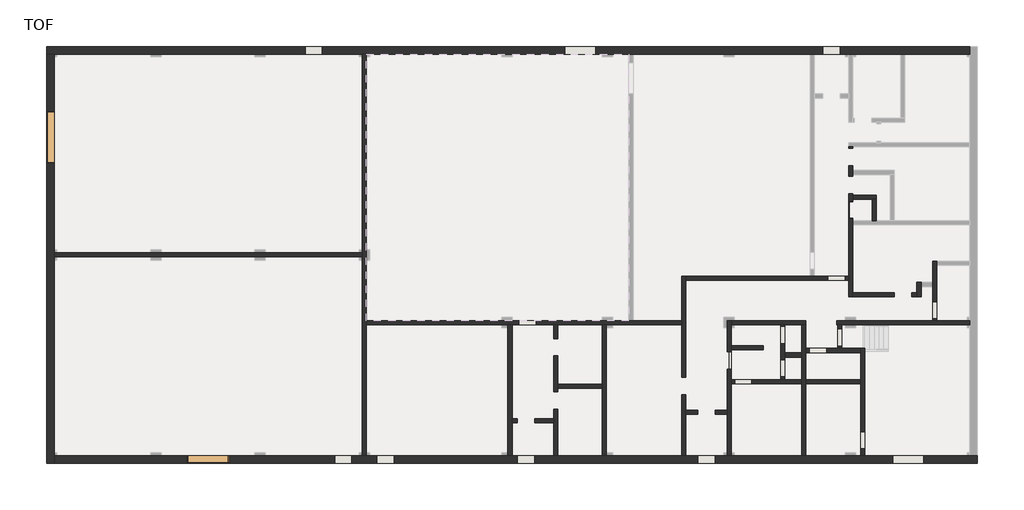
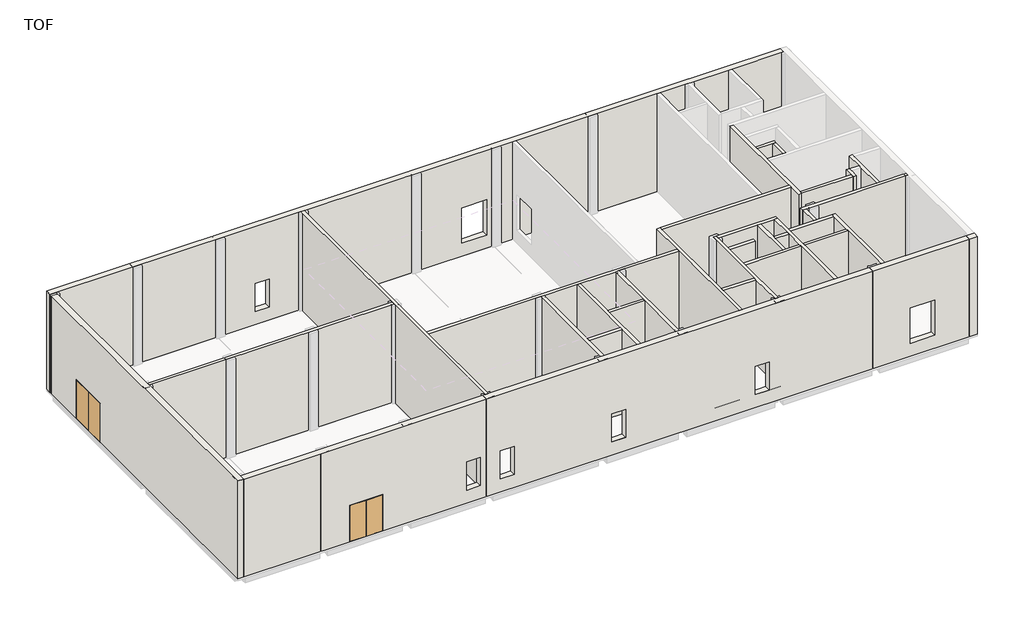
# One storey, part 1 of 3: 31 walls, 3 doors.
"""IFC4 building model written with IfcOpenShell, lengths in millimetres."""

import ifcopenshell
import ifcopenshell.guid

model = None  # the IFC model being written
_history = None  # IfcOwnerHistory: only IFC2X3 demands one
_inside = {}  # id of a spatial element -> (the spatial element, [elements in it])
_under = {}  # id of a project, library or spatial element -> (it, [spatial elements below it])
_declared = {}  # id of a project -> (the project, [libraries it declares])
_typed = {}  # id of a type object -> (the type object, [elements of that type])
_made_of = {}  # id of a material, layer set ... -> (it, [elements and type objects made of it])


def new_model(schema):
    """Start an empty IFC model of exactly this schema.

    Asked for "IFC4X3", IfcOpenShell would pick the latest addendum, in which some entities
    have other attributes; the version numbers below select the first issue.
    IFC2X3 requires an IfcOwnerHistory on every rooted entity: one is made here for all.
    """
    global model, _history
    if schema == "IFC4X3":
        model = ifcopenshell.file(schema_version=(4, 3, 0, 0))
    else:
        model = ifcopenshell.file(schema=schema)
    _inside.clear()
    _under.clear()
    _declared.clear()
    _typed.clear()
    _made_of.clear()
    _history = None
    if model.schema == "IFC2X3":
        org = make("IfcOrganization", Name="unknown")
        user = make(
            "IfcPersonAndOrganization",
            ThePerson=make("IfcPerson", FamilyName="unknown"),
            TheOrganization=org,
        )
        app = make(
            "IfcApplication",
            ApplicationDeveloper=org,
            Version="unknown",
            ApplicationFullName="unknown",
            ApplicationIdentifier="unknown",
        )
        _history = make(
            "IfcOwnerHistory",
            OwningUser=user,
            OwningApplication=app,
            ChangeAction="ADDED",
            CreationDate=0,
        )
    return model


def make(cls, **values):
    """One entity of the class cls with the attributes given. An attribute that is None is left unset."""
    return model.create_entity(
        cls, **{name: value for name, value in values.items() if value is not None}
    )


def rooted(cls, **values):
    """An entity with a GlobalId (a new one), such as an element, a storey or a relation."""
    return make(cls, GlobalId=ifcopenshell.guid.new(), OwnerHistory=_history, **values)


def si_unit(unit_type, name, prefix=None):
    """IfcSIUnit, for example si_unit("LENGTHUNIT", "METRE", prefix="MILLI")."""
    return make("IfcSIUnit", UnitType=unit_type, Prefix=prefix, Name=name)


def assignment(units):
    """IfcUnitAssignment: the units of a project."""
    return None if units is None else make("IfcUnitAssignment", Units=units)


def point(xyz):
    """IfcCartesianPoint."""
    return None if xyz is None else make("IfcCartesianPoint", Coordinates=xyz)


def direction(xyz):
    """IfcDirection."""
    return None if xyz is None else make("IfcDirection", DirectionRatios=xyz)


def frame(location, z_axis=None, x_axis=None):
    """IfcAxis2Placement3D, a coordinate frame: its origin and axes. An axis left out is left unset."""
    return make(
        "IfcAxis2Placement3D",
        Location=point(location),
        Axis=direction(z_axis),
        RefDirection=direction(x_axis),
    )


def origin():
    """The frame at (0, 0, 0) with its axes left unset."""
    return frame((0.0, 0.0, 0.0))


def place(relative_to, where):
    """IfcLocalPlacement: puts the frame where relative to a parent placement (None: the world)."""
    return make(
        "IfcLocalPlacement", PlacementRelTo=relative_to, RelativePlacement=where
    )


def context(
    kind, dimensions, precision=None, world=None, true_north=None, identifier=None
):
    """IfcGeometricRepresentationContext, for example the 3D "Model" context."""
    return make(
        "IfcGeometricRepresentationContext",
        ContextIdentifier=identifier,
        ContextType=kind,
        CoordinateSpaceDimension=dimensions,
        Precision=precision,
        WorldCoordinateSystem=world,
        TrueNorth=true_north,
    )


def project(units=None, contexts=None):
    """IfcProject with its units and contexts."""
    return rooted(
        "IfcProject",
        Name="project",
        RepresentationContexts=contexts,
        UnitsInContext=assignment(units),
    )


def spatial(cls, under=None, at=None, **own):
    """A site, building, storey or space (cls), placed at a placement, below another one or the project."""
    s = rooted(cls, ObjectPlacement=at, **own)
    if under is not None:
        _under.setdefault(under.id(), (under, []))[1].append(s)
    return s


def polyline(points):
    """IfcPolyline through the points."""
    return make("IfcPolyline", Points=[point(p) for p in points])


def outline(outer, holes=None, kind="AREA"):
    """IfcArbitraryClosedProfileDef: a profile drawn as a closed curve; with holes, ...WithVoids."""
    if holes is None:
        return make("IfcArbitraryClosedProfileDef", ProfileType=kind, OuterCurve=outer)
    return make(
        "IfcArbitraryProfileDefWithVoids",
        ProfileType=kind,
        OuterCurve=outer,
        InnerCurves=holes,
    )


def extrude(swept, where, along, depth):
    """IfcExtrudedAreaSolid: the profile swept, set in the frame where, extruded along a direction by depth."""
    return make(
        "IfcExtrudedAreaSolid",
        SweptArea=swept,
        Position=where,
        ExtrudedDirection=direction(along),
        Depth=depth,
    )


def faces_of(points, faces, orient=None, outer=None):
    """IfcFace entities. A face is a list of loops; a loop is a list of indices into points, from 0.

    orient and outer hold one flag for each loop. By default every Orientation is true, the
    first loop of a face is its IfcFaceOuterBound and the others are IfcFaceBound.
    """
    made = []
    for i, loops in enumerate(faces):
        bounds = []
        for j, loop in enumerate(loops):
            is_outer = j == 0 if outer is None else outer[i][j]
            bounds.append(
                make(
                    "IfcFaceOuterBound" if is_outer else "IfcFaceBound",
                    Bound=make("IfcPolyLoop", Polygon=[points[k] for k in loop]),
                    Orientation=True if orient is None else orient[i][j],
                )
            )
        made.append(make("IfcFace", Bounds=bounds))
    return made


def faceted_brep(points, faces, orient=None, outer=None, voids=None):
    """IfcFacetedBrep: a solid bounded by flat faces; with voids (closed shells), ...WithVoids."""
    shared = [point(p) for p in points]
    hull = make("IfcClosedShell", CfsFaces=faces_of(shared, faces, orient, outer))
    if voids is None:
        return make("IfcFacetedBrep", Outer=hull)
    return make(
        "IfcFacetedBrepWithVoids",
        Outer=hull,
        Voids=[
            make(cls, CfsFaces=faces_of(shared, fs, o, b)) for cls, fs, o, b in voids
        ],
    )


def shape(context_of_items, identifier, shape_type, items):
    """IfcShapeRepresentation: the items that make up one representation, for example the "Body"."""
    return make(
        "IfcShapeRepresentation",
        ContextOfItems=context_of_items,
        RepresentationIdentifier=identifier,
        RepresentationType=shape_type,
        Items=items,
    )


def source(mapping_origin, context_of_items, identifier, shape_type, items):
    """IfcRepresentationMap: a shape defined once, which mapped items show again and again."""
    return make(
        "IfcRepresentationMap",
        MappingOrigin=mapping_origin,
        MappedRepresentation=shape(context_of_items, identifier, shape_type, items),
    )


def transform(
    local_origin,
    x_axis=None,
    y_axis=None,
    z_axis=None,
    scale=None,
    scale2=None,
    scale3=None,
    uniform=True,
):
    """IfcCartesianTransformationOperator3D, or its non-uniform kind. x_axis, y_axis, z_axis: its Axis1, 2, 3."""
    if uniform:
        return make(
            "IfcCartesianTransformationOperator3D",
            Axis1=direction(x_axis),
            Axis2=direction(y_axis),
            LocalOrigin=point(local_origin),
            Scale=scale,
            Axis3=direction(z_axis),
        )
    return make(
        "IfcCartesianTransformationOperator3DnonUniform",
        Axis1=direction(x_axis),
        Axis2=direction(y_axis),
        LocalOrigin=point(local_origin),
        Scale=scale,
        Axis3=direction(z_axis),
        Scale2=scale2,
        Scale3=scale3,
    )


def mapped(mapping_source, mapping_target):
    """IfcMappedItem: shows the shape of a source again, moved by a transform."""
    return make(
        "IfcMappedItem", MappingSource=mapping_source, MappingTarget=mapping_target
    )


def made_of(thing, what):
    """Note that an element or type object is made of a material, layer set ...; save() writes the relation."""
    if what is not None:
        _made_of.setdefault(what.id(), (what, []))[1].append(thing)
    return thing


def element(
    cls,
    number,
    at=None,
    inside=None,
    cuts=None,
    type_object=None,
    material=None,
    context=None,
    identifier="Body",
    shape_type=None,
    held_by="IfcProductDefinitionShape",
    body=None,
    shapes=None,
    **own,
):
    """One element of the class cls, such as IfcWall. Its Tag is "e" and its number.

    at: its placement. inside: the storey or other place that contains it. cuts: it is an
    opening in that element (IfcRelVoidsElement). A single representation is given by context,
    identifier, shape_type and body (its items); several are given by shapes. held_by: the class
    of the entity that holds the representations. save() writes the other relations.
    """
    e = rooted(cls, Tag="e%d" % number, ObjectPlacement=at, **own)
    if body is not None:
        shapes = [shape(context, identifier, shape_type, body)]
    if shapes is not None:
        e.Representation = make(held_by, Representations=shapes)
    if inside is not None:
        _inside.setdefault(inside.id(), (inside, []))[1].append(e)
    if cuts is not None:
        rooted(
            "IfcRelVoidsElement", RelatingBuildingElement=cuts, RelatedOpeningElement=e
        )
    if type_object is not None:
        _typed.setdefault(type_object.id(), (type_object, []))[1].append(e)
    return made_of(e, material)


def aggregate(whole, parts):
    """IfcRelAggregates: a whole, such as a stair, and the parts it consists of."""
    return rooted("IfcRelAggregates", RelatingObject=whole, RelatedObjects=parts)


def save(model, path):
    """Write the relations noted so far, then the file.

    IfcRelAggregates (storeys below a building ...), IfcRelContainedInSpatialStructure (elements
    in a storey), IfcRelDefinesByType, IfcRelAssociatesMaterial and IfcRelDeclares: one each for
    every whole, place, type object, material and project.
    """
    for whole, parts in _under.values():
        aggregate(whole, parts)
    for where, things in _inside.values():
        rooted(
            "IfcRelContainedInSpatialStructure",
            RelatedElements=things,
            RelatingStructure=where,
        )
    for kind, things in _typed.values():
        rooted("IfcRelDefinesByType", RelatedObjects=things, RelatingType=kind)
    for what, things in _made_of.values():
        rooted("IfcRelAssociatesMaterial", RelatedObjects=things, RelatingMaterial=what)
    for by, libraries in _declared.values():
        rooted("IfcRelDeclares", RelatingContext=by, RelatedDefinitions=libraries)
    model.write(path)


def double_door_steel_89dfd0fe(model_context):
    return source(origin(), model_context, "Body", "SolidModel", [
        extrude(outline(polyline([(1480.0, 175.0), (0.0, 175.0), (0.0, 215.0), (1480.0, 215.0), (1480.0, 175.0)])), frame((0.0, 0.0, 20.0), z_axis=(0.0, 0.0, 1.0), x_axis=(1.0, 0.0, 0.0)), (0.0, 0.0, 1.0), 2960.0),
        extrude(outline(polyline([(0.0, 175.0), (-1480.0, 175.0), (-1480.0, 215.0), (0.0, 215.0), (0.0, 175.0)])), frame((0.0, 0.0, 20.0), z_axis=(0.0, 0.0, 1.0), x_axis=(1.0, 0.0, 0.0)), (0.0, 0.0, 1.0), 2960.0),
        faceted_brep([(1500.0, -215.0, 3000.0), (1500.0, 215.0, 3000.0), (-1500.0, 215.0, 3000.0), (-1500.0, -215.0, 3000.0), (1465.0, 175.0, 2965.0), (1465.0, -215.0, 2965.0), (-1465.0, -215.0, 2965.0), (-1465.0, 175.0, 2965.0), (1480.0, 215.0, 2980.0), (1480.0, 175.0, 2980.0), (-1480.0, 175.0, 2980.0), (-1480.0, 215.0, 2980.0), (-1500.0, 215.0, 0.0), (-1500.0, -215.0, 0.0), (-1465.0, -215.0, 35.0), (-1465.0, 175.0, 35.0), (-1480.0, 175.0, 20.0), (-1480.0, 215.0, 20.0), (1500.0, 215.0, 0.0), (1480.0, 215.0, 20.0), (1500.0, -215.0, 0.0), (1465.0, -215.0, 35.0), (1465.0, 175.0, 35.0), (1480.0, 175.0, 20.0)], [[[0, 1, 2, 3]], [[4, 5, 6, 7]], [[8, 9, 10, 11]], [[3, 2, 12, 13]], [[7, 6, 14, 15]], [[11, 10, 16, 17]], [[18, 12, 2, 1], [8, 11, 17, 19]], [[13, 12, 18, 20]], [[0, 3, 13, 20], [21, 14, 6, 5]], [[15, 14, 21, 22]], [[23, 16, 10, 9], [4, 7, 15, 22]], [[17, 16, 23, 19]], [[20, 18, 1, 0]], [[22, 21, 5, 4]], [[19, 23, 9, 8]]]),
    ])


def double_door_steel_f76c4a76(model_context):
    return source(origin(), model_context, "Body", "SolidModel", [
        extrude(outline(polyline([(1180.0, 175.0), (0.0, 175.0), (0.0, 215.0), (1180.0, 215.0), (1180.0, 175.0)])), frame((0.0, 0.0, 20.0), z_axis=(0.0, 0.0, 1.0), x_axis=(1.0, 0.0, 0.0)), (0.0, 0.0, 1.0), 2760.0),
        extrude(outline(polyline([(0.0, 175.0), (-1180.0, 175.0), (-1180.0, 215.0), (0.0, 215.0), (0.0, 175.0)])), frame((0.0, 0.0, 20.0), z_axis=(0.0, 0.0, 1.0), x_axis=(1.0, 0.0, 0.0)), (0.0, 0.0, 1.0), 2760.0),
        faceted_brep([(1200.0, -215.0, 0.0), (1200.0, 215.0, 0.0), (1200.0, 215.0, 2800.0), (1200.0, -215.0, 2800.0), (-1200.0, 215.0, 2800.0), (-1200.0, -215.0, 2800.0), (-1200.0, 215.0, 0.0), (1180.0, 215.0, 2780.0), (-1180.0, 215.0, 2780.0), (-1180.0, 215.0, 20.0), (1180.0, 215.0, 20.0), (-1200.0, -215.0, 0.0), (1165.0, -215.0, 35.0), (-1165.0, -215.0, 35.0), (-1165.0, -215.0, 2765.0), (1165.0, -215.0, 2765.0), (1165.0, 175.0, 35.0), (1165.0, 175.0, 2765.0), (-1165.0, 175.0, 2765.0), (-1165.0, 175.0, 35.0), (1180.0, 175.0, 20.0), (-1180.0, 175.0, 20.0), (-1180.0, 175.0, 2780.0), (1180.0, 175.0, 2780.0)], [[[0, 1, 2, 3]], [[3, 2, 4, 5]], [[1, 6, 4, 2], [7, 8, 9, 10]], [[5, 4, 6, 11]], [[3, 5, 11, 0], [12, 13, 14, 15]], [[16, 12, 15, 17]], [[17, 15, 14, 18]], [[18, 14, 13, 19]], [[20, 21, 22, 23], [17, 18, 19, 16]], [[10, 20, 23, 7]], [[7, 23, 22, 8]], [[8, 22, 21, 9]], [[11, 6, 1, 0]], [[19, 13, 12, 16]], [[9, 21, 20, 10]]]),
    ])


def double_door_steel_898613e4(model_context):
    return source(origin(), model_context, "Body", "SolidModel", [
        extrude(outline(polyline([(480.0, 77.0), (0.0, 77.0), (0.0, 117.0), (480.0, 117.0), (480.0, 77.0)])), frame((0.0, 0.0, 20.0), z_axis=(0.0, 0.0, 1.0), x_axis=(1.0, 0.0, 0.0)), (0.0, 0.0, 1.0), 2110.0),
        extrude(outline(polyline([(0.0, 77.0), (-480.0, 77.0), (-480.0, 117.0), (0.0, 117.0), (0.0, 77.0)])), frame((0.0, 0.0, 20.0), z_axis=(0.0, 0.0, 1.0), x_axis=(1.0, 0.0, 0.0)), (0.0, 0.0, 1.0), 2110.0),
        faceted_brep([(500.0, -117.0, 0.0), (500.0, 117.0, 0.0), (500.0, 117.0, 2150.0), (500.0, -117.0, 2150.0), (-500.0, 117.0, 2150.0), (-500.0, -117.0, 2150.0), (-500.0, 117.0, 0.0), (480.0, 117.0, 2130.0), (-480.0, 117.0, 2130.0), (-480.0, 117.0, 20.0), (480.0, 117.0, 20.0), (-500.0, -117.0, 0.0), (465.0, -117.0, 35.0), (-465.0, -117.0, 35.0), (-465.0, -117.0, 2115.0), (465.0, -117.0, 2115.0), (465.0, 77.0, 35.0), (465.0, 77.0, 2115.0), (-465.0, 77.0, 2115.0), (-465.0, 77.0, 35.0), (480.0, 77.0, 20.0), (-480.0, 77.0, 20.0), (-480.0, 77.0, 2130.0), (480.0, 77.0, 2130.0)], [[[0, 1, 2, 3]], [[3, 2, 4, 5]], [[1, 6, 4, 2], [7, 8, 9, 10]], [[5, 4, 6, 11]], [[3, 5, 11, 0], [12, 13, 14, 15]], [[16, 12, 15, 17]], [[17, 15, 14, 18]], [[18, 14, 13, 19]], [[20, 21, 22, 23], [17, 18, 19, 16]], [[10, 20, 23, 7]], [[7, 23, 22, 8]], [[8, 22, 21, 9]], [[11, 6, 1, 0]], [[19, 13, 12, 16]], [[9, 21, 20, 10]]]),
    ])


model = new_model("IFC4")

# Units and contexts
model_context = context("Model", 3, world=origin())
ifc_project = project(units=[si_unit("LENGTHUNIT", "METRE", prefix="MILLI")], contexts=[model_context])

# Site, building, storey
site = spatial("IfcSite", under=ifc_project)
building = spatial("IfcBuilding", under=site)
storey = spatial("IfcBuildingStorey", under=building, Name="TOF", Elevation=150.0)

# Doors
placement = place(None, origin())
double_door_steel_shape = double_door_steel_89dfd0fe(model_context)
element("IfcDoor", 1, ObjectType="Double Door_Steel : H_DR_AMB_Double Door_Steel_W3000xH3000", at=placement, inside=storey, context=model_context, shape_type="MappedRepresentation", body=[
    mapped(double_door_steel_shape, transform((-160.3, 19086.5208589, 150.0), x_axis=(0.0, 1.0, 0.0), y_axis=(-1.0, 0.0, 0.0), z_axis=(0.0, 0.0, 1.0))),
])
double_door_steel_2_shape = double_door_steel_f76c4a76(model_context)
element("IfcDoor", 2, ObjectType="Double Door_Steel : H_DR_AMB_Double Door_Steel_W2400xH2800", at=placement, inside=storey, context=model_context, shape_type="MappedRepresentation", body=[
    mapped(double_door_steel_2_shape, transform((8931.2, 531.5208589, 150.0), x_axis=(-1.0, 0.0, 0.0), y_axis=(0.0, -1.0, 0.0), z_axis=(0.0, 0.0, 1.0))),
])
double_door_steel_3_shape = double_door_steel_898613e4(model_context)
element("IfcDoor", 3, ObjectType="Double Door_Steel : H_DR_AMB_Double Door_Steel_W1000xH2150", at=placement, inside=storey, context=model_context, shape_type="MappedRepresentation", body=[
    mapped(double_door_steel_3_shape, transform((45924.7, 14901.8721317, 150.0), x_axis=(0.0, 1.0, 0.0), y_axis=(-1.0, 0.0, 0.0), z_axis=(0.0, 0.0, 1.0))),
])

# Walls
element("IfcWall", 4, ObjectType="H_WA_AMW_Brick Wall_Ext (0.5B_50_1.0B / Emulsion)", at=placement, inside=storey, context=model_context, shape_type="Brep", body=[
    faceted_brep([(-375.3, 23886.5208589, 150.0), (54.7, 23886.5208589, 150.0), (17807.7, 23886.5208589, 150.0), (18041.7, 23886.5208589, 150.0), (33157.7, 23886.5208589, 150.0), (33391.7, 23886.5208589, 150.0), (43607.7, 23886.5208589, 150.0), (43841.7, 23886.5208589, 150.0), (52794.7, 23886.5208589, 150.0), (52794.7, 23886.5208589, 7650.0), (49041.7, 23886.5208589, 7650.0), (48807.7, 23886.5208589, 7650.0), (46041.7, 23886.5208589, 7650.0), (45807.7, 23886.5208589, 7650.0), (43841.7, 23886.5208589, 7650.0), (43607.7, 23886.5208589, 7650.0), (33391.7, 23886.5208589, 7650.0), (33157.7, 23886.5208589, 7650.0), (18041.7, 23886.5208589, 7650.0), (17807.7, 23886.5208589, 7650.0), (54.7, 23886.5208589, 7650.0), (-375.3, 23886.5208589, 7650.0), (14507.7, 23886.5208589, 1150.0), (14507.7, 23886.5208589, 3300.0), (15507.7, 23886.5208589, 3300.0), (15507.7, 23886.5208589, 1150.0), (31257.7, 23886.5208589, 3850.0), (31257.7, 23886.5208589, 1150.0), (29457.7, 23886.5208589, 1150.0), (29457.7, 23886.5208589, 3850.0), (44324.7, 23886.5208589, 1150.0), (44324.7, 23886.5208589, 3300.0), (45324.7, 23886.5208589, 3300.0), (45324.7, 23886.5208589, 1150.0), (52794.7, 24316.5208589, 150.0), (-375.3, 24316.5208589, 150.0), (-375.3, 24316.5208589, 7650.0), (52794.7, 24316.5208589, 7650.0), (14507.7, 24316.5208589, 3300.0), (14507.7, 24316.5208589, 1150.0), (15507.7, 24316.5208589, 1150.0), (15507.7, 24316.5208589, 3300.0), (31257.7, 24316.5208589, 1150.0), (31257.7, 24316.5208589, 3850.0), (29457.7, 24316.5208589, 3850.0), (29457.7, 24316.5208589, 1150.0), (44324.7, 24316.5208589, 3300.0), (44324.7, 24316.5208589, 1150.0), (45324.7, 24316.5208589, 1150.0), (45324.7, 24316.5208589, 3300.0)], [[[0, 1, 2, 3, 4, 5, 6, 7, 8, 9, 10, 11, 12, 13, 14, 15, 16, 17, 18, 19, 20, 21], [22, 23, 24, 25], [26, 27, 28, 29], [30, 31, 32, 33]], [[34, 35, 36, 37], [38, 39, 40, 41], [42, 43, 44, 45], [46, 47, 48, 49]], [[8, 7, 6, 5, 4, 3, 2, 1, 0, 35, 34]], [[21, 20, 19, 18, 17, 16, 15, 14, 13, 12, 11, 10, 9, 37, 36]], [[0, 21, 36, 35]], [[9, 8, 34, 37]], [[22, 39, 38, 23]], [[23, 38, 41, 24]], [[24, 41, 40, 25]], [[39, 22, 25, 40]], [[42, 27, 26, 43]], [[43, 26, 29, 44]], [[28, 45, 44, 29]], [[27, 42, 45, 28]], [[31, 30, 47, 46]], [[32, 31, 46, 49]], [[33, 32, 49, 48]], [[30, 33, 48, 47]]]),
])
element("IfcWall", 5, ObjectType="H_WA_AMW_Brick Wall_Ext (0.5B_50_1.0B / Emulsion)", at=placement, inside=storey, context=model_context, shape_type="Brep", body=[
    faceted_brep([(54.7, 23886.5208589, 7650.0), (54.7, 12433.5208589, 7650.0), (54.7, 12199.5208589, 7650.0), (54.7, 746.5208589, 7650.0), (54.7, 316.5208589, 7650.0), (54.7, 316.5208589, 150.0), (54.7, 746.5208589, 150.0), (54.7, 12199.5208589, 150.0), (54.7, 12433.5208589, 150.0), (54.7, 17586.5208589, 150.0), (54.7, 17586.5208589, 3150.0), (54.7, 20586.5208589, 3150.0), (54.7, 20586.5208589, 150.0), (54.7, 23886.5208589, 150.0), (-375.3, 316.5208589, 7650.0), (-375.3, 23886.5208589, 7650.0), (-375.3, 23886.5208589, 150.0), (-375.3, 20586.5208589, 150.0), (-375.3, 20586.5208589, 3150.0), (-375.3, 17586.5208589, 3150.0), (-375.3, 17586.5208589, 150.0), (-375.3, 316.5208589, 150.0)], [[[0, 1, 2, 3, 4, 5, 6, 7, 8, 9, 10, 11, 12, 13]], [[14, 15, 16, 17, 18, 19, 20, 21]], [[5, 21, 20, 9, 8, 7, 6]], [[16, 13, 12, 17]], [[4, 3, 2, 1, 0, 15, 14]], [[5, 4, 14, 21]], [[0, 13, 16, 15]], [[11, 18, 17, 12]], [[18, 11, 10, 19]], [[19, 10, 9, 20]]]),
])
element("IfcWall", 6, ObjectType="H_WA_AMW_Brick Wall_Ext (0.5B_50_1.0B / Emulsion)", at=placement, inside=storey, context=model_context, shape_type="Brep", body=[
    faceted_brep([(54.7, 746.5208589, 7650.0), (17807.7, 746.5208589, 7650.0), (18041.7, 746.5208589, 7650.0), (26190.7, 746.5208589, 7650.0), (26424.7, 746.5208589, 7650.0), (28824.7, 746.5208589, 7650.0), (29058.7, 746.5208589, 7650.0), (31624.7, 746.5208589, 7650.0), (31858.7, 746.5208589, 7650.0), (36207.7, 746.5208589, 7650.0), (36441.7, 746.5208589, 7650.0), (38807.7, 746.5208589, 7650.0), (39041.7, 746.5208589, 7650.0), (43107.7, 746.5208589, 7650.0), (43341.7, 746.5208589, 7650.0), (46507.7, 746.5208589, 7650.0), (46741.7, 746.5208589, 7650.0), (52794.7, 746.5208589, 7650.0), (53224.7, 746.5208589, 7650.0), (53224.7, 746.5208589, 150.0), (52794.7, 746.5208589, 150.0), (46741.7, 746.5208589, 150.0), (46507.7, 746.5208589, 150.0), (43341.7, 746.5208589, 150.0), (43107.7, 746.5208589, 150.0), (39041.7, 746.5208589, 150.0), (38807.7, 746.5208589, 150.0), (26424.7, 746.5208589, 150.0), (26190.7, 746.5208589, 150.0), (18041.7, 746.5208589, 150.0), (17807.7, 746.5208589, 150.0), (10131.2, 746.5208589, 150.0), (10131.2, 746.5208589, 2950.0), (7731.2, 746.5208589, 2950.0), (7731.2, 746.5208589, 150.0), (54.7, 746.5208589, 150.0), (16207.7, 746.5208589, 3300.0), (16207.7, 746.5208589, 1150.0), (17207.7, 746.5208589, 1150.0), (17207.7, 746.5208589, 3300.0), (19641.7, 746.5208589, 1150.0), (19641.7, 746.5208589, 3300.0), (18641.7, 746.5208589, 3300.0), (18641.7, 746.5208589, 1150.0), (27724.7, 746.5208589, 1150.0), (27724.7, 746.5208589, 3300.0), (26724.7, 746.5208589, 3300.0), (26724.7, 746.5208589, 1150.0), (37124.7, 746.5208589, 3300.0), (37124.7, 746.5208589, 1150.0), (38124.7, 746.5208589, 1150.0), (38124.7, 746.5208589, 3300.0), (48341.7, 746.5208589, 3850.0), (48341.7, 746.5208589, 1150.0), (50141.7, 746.5208589, 1150.0), (50141.7, 746.5208589, 3850.0), (53224.7, 316.5208589, 7650.0), (54.7, 316.5208589, 7650.0), (54.7, 316.5208589, 150.0), (7731.2, 316.5208589, 150.0), (7731.2, 316.5208589, 2950.0), (10131.2, 316.5208589, 2950.0), (10131.2, 316.5208589, 150.0), (53224.7, 316.5208589, 150.0), (16207.7, 316.5208589, 1150.0), (16207.7, 316.5208589, 3300.0), (17207.7, 316.5208589, 3300.0), (17207.7, 316.5208589, 1150.0), (19641.7, 316.5208589, 3300.0), (19641.7, 316.5208589, 1150.0), (18641.7, 316.5208589, 1150.0), (18641.7, 316.5208589, 3300.0), (27724.7, 316.5208589, 3300.0), (27724.7, 316.5208589, 1150.0), (26724.7, 316.5208589, 1150.0), (26724.7, 316.5208589, 3300.0), (37124.7, 316.5208589, 1150.0), (37124.7, 316.5208589, 3300.0), (38124.7, 316.5208589, 3300.0), (38124.7, 316.5208589, 1150.0), (48341.7, 316.5208589, 1150.0), (48341.7, 316.5208589, 3850.0), (50141.7, 316.5208589, 3850.0), (50141.7, 316.5208589, 1150.0)], [[[0, 1, 2, 3, 4, 5, 6, 7, 8, 9, 10, 11, 12, 13, 14, 15, 16, 17, 18, 19, 20, 21, 22, 23, 24, 25, 26, 27, 28, 29, 30, 31, 32, 33, 34, 35], [36, 37, 38, 39], [40, 41, 42, 43], [44, 45, 46, 47], [48, 49, 50, 51], [52, 53, 54, 55]], [[56, 57, 58, 59, 60, 61, 62, 63], [64, 65, 66, 67], [68, 69, 70, 71], [72, 73, 74, 75], [76, 77, 78, 79], [80, 81, 82, 83]], [[19, 63, 62, 31, 30, 29, 28, 27, 26, 25, 24, 23, 22, 21, 20]], [[58, 35, 34, 59]], [[18, 17, 16, 15, 14, 13, 12, 11, 10, 9, 8, 7, 6, 5, 4, 3, 2, 1, 0, 57, 56]], [[19, 18, 56, 63]], [[0, 35, 58, 57]], [[33, 60, 59, 34]], [[60, 33, 32, 61]], [[61, 32, 31, 62]], [[64, 37, 36, 65]], [[65, 36, 39, 66]], [[66, 39, 38, 67]], [[37, 64, 67, 38]], [[41, 40, 69, 68]], [[42, 41, 68, 71]], [[43, 42, 71, 70]], [[40, 43, 70, 69]], [[45, 44, 73, 72]], [[46, 45, 72, 75]], [[47, 46, 75, 74]], [[44, 47, 74, 73]], [[76, 49, 48, 77]], [[77, 48, 51, 78]], [[50, 79, 78, 51]], [[49, 76, 79, 50]], [[80, 53, 52, 81]], [[81, 52, 55, 82]], [[54, 83, 82, 55]], [[53, 80, 83, 54]]]),
])
element("IfcWall", 7, ObjectType="H_WA_AMW_Block Wall_Int_T200 (Both Plaster_Emulsion)", at=placement, inside=storey, context=model_context, shape_type="SweptSolid", body=[
    extrude(outline(polyline([(17807.7, 12199.5208589), (54.7, 12199.5208589), (54.7, 12433.5208589), (17807.7, 12433.5208589), (17807.7, 12199.5208589)])), frame((0.0, 0.0, 150.0), z_axis=(0.0, 0.0, 1.0), x_axis=(1.0, 0.0, 0.0)), (0.0, 0.0, 1.0), 7500.0),
])
element("IfcWall", 8, ObjectType="H_WA_AMW_Block Wall_Int_T200 (Both Plaster_Emulsion)", at=placement, inside=storey, context=model_context, shape_type="Brep", body=[
    faceted_brep([(17807.7, 23886.5208589, 150.0), (17807.7, 12433.5208589, 150.0), (17807.7, 12199.5208589, 150.0), (17807.7, 746.5208589, 150.0), (17807.7, 746.5208589, 7650.0), (17807.7, 12199.5208589, 7650.0), (17807.7, 12433.5208589, 7650.0), (17807.7, 23886.5208589, 7650.0), (18041.7, 23886.5208589, 150.0), (18041.7, 23886.5208589, 7650.0), (18041.7, 8533.5208589, 7650.0), (18041.7, 8299.5208589, 7650.0), (18041.7, 746.5208589, 7650.0), (18041.7, 746.5208589, 150.0), (18041.7, 8299.5208589, 150.0), (18041.7, 8533.5208589, 150.0)], [[[0, 1, 2, 3, 4, 5, 6, 7]], [[8, 9, 10, 11, 12, 13, 14, 15]], [[3, 2, 1, 0, 8, 15, 14, 13]], [[7, 6, 5, 4, 12, 11, 10, 9]], [[0, 7, 9, 8]], [[4, 3, 13, 12]]]),
])
element("IfcWall", 9, ObjectType="H_WA_AMW_Block Wall_Int_T200 (Both Plaster_Emulsion)", at=placement, inside=storey, context=model_context, shape_type="Brep", body=[
    faceted_brep([(18041.7, 8299.5208589, 150.0), (26190.7, 8299.5208589, 150.0), (26424.7, 8299.5208589, 150.0), (36207.7, 8299.5208589, 150.0), (36207.7, 8299.5208589, 7650.0), (31858.7, 8299.5208589, 7650.0), (31624.7, 8299.5208589, 7650.0), (29058.7, 8299.5208589, 7650.0), (28824.7, 8299.5208589, 7650.0), (26424.7, 8299.5208589, 7650.0), (26190.7, 8299.5208589, 7650.0), (18041.7, 8299.5208589, 7650.0), (27824.7, 8299.5208589, 3300.0), (27824.7, 8299.5208589, 1150.0), (26824.7, 8299.5208589, 1150.0), (26824.7, 8299.5208589, 3300.0), (36207.7, 8533.5208589, 150.0), (33391.7, 8533.5208589, 150.0), (33157.7, 8533.5208589, 150.0), (18041.7, 8533.5208589, 150.0), (18041.7, 8533.5208589, 7650.0), (33157.7, 8533.5208589, 7650.0), (33391.7, 8533.5208589, 7650.0), (36207.7, 8533.5208589, 7650.0), (27824.7, 8533.5208589, 1150.0), (27824.7, 8533.5208589, 3300.0), (26824.7, 8533.5208589, 3300.0), (26824.7, 8533.5208589, 1150.0)], [[[0, 1, 2, 3, 4, 5, 6, 7, 8, 9, 10, 11], [12, 13, 14, 15]], [[16, 17, 18, 19, 20, 21, 22, 23], [24, 25, 26, 27]], [[3, 2, 1, 0, 19, 18, 17, 16]], [[11, 10, 9, 8, 7, 6, 5, 4, 23, 22, 21, 20]], [[0, 11, 20, 19]], [[4, 3, 16, 23]], [[24, 13, 12, 25]], [[25, 12, 15, 26]], [[26, 15, 14, 27]], [[13, 24, 27, 14]]]),
])
element("IfcWall", 10, ObjectType="H_WA_AMW_Block Wall_Int_T200 (Both Plaster_Emulsion)", at=placement, inside=storey, context=model_context, shape_type="Brep", body=[
    faceted_brep([(36207.7, 746.5208589, 7650.0), (36207.7, 8299.5208589, 7650.0), (36207.7, 8533.5208589, 7650.0), (36207.7, 11083.5208589, 7650.0), (36207.7, 11083.5208589, 1150.0), (36207.7, 5280.5208589, 1150.0), (36207.7, 5280.5208589, 3300.0), (36207.7, 4280.5208589, 3300.0), (36207.7, 4280.5208589, 1150.0), (36207.7, 746.5208589, 1150.0), (36441.7, 11083.5208589, 7650.0), (36441.7, 10849.5208589, 7650.0), (36441.7, 3380.5208589, 7650.0), (36441.7, 3146.5208589, 7650.0), (36441.7, 746.5208589, 7650.0), (36441.7, 746.5208589, 1150.0), (36441.7, 3146.5208589, 1150.0), (36441.7, 3380.5208589, 1150.0), (36441.7, 4280.5208589, 1150.0), (36441.7, 4280.5208589, 3300.0), (36441.7, 5280.5208589, 3300.0), (36441.7, 5280.5208589, 1150.0), (36441.7, 11083.5208589, 1150.0)], [[[0, 1, 2, 3, 4, 5, 6, 7, 8, 9]], [[10, 11, 12, 13, 14, 15, 16, 17, 18, 19, 20, 21, 22]], [[15, 9, 8, 18, 17, 16]], [[4, 22, 21, 5]], [[3, 2, 1, 0, 14, 13, 12, 11, 10]], [[0, 9, 15, 14]], [[4, 3, 10, 22]], [[20, 6, 5, 21]], [[6, 20, 19, 7]], [[7, 19, 18, 8]]]),
])
element("IfcWall", 11, ObjectType="H_WA_AMW_Block Wall_Int_T200 (Both Plaster_Emulsion)", at=placement, inside=storey, context=model_context, shape_type="Brep", body=[
    faceted_brep([(36441.7, 10849.5208589, 150.0), (45807.7, 10849.5208589, 150.0), (45807.7, 10849.5208589, 7650.0), (36441.7, 10849.5208589, 7650.0), (44607.7, 10849.5208589, 1150.0), (44607.7, 10849.5208589, 3300.0), (45607.7, 10849.5208589, 3300.0), (45607.7, 10849.5208589, 1150.0), (45807.7, 11083.5208589, 150.0), (43841.7, 11083.5208589, 150.0), (43607.7, 11083.5208589, 150.0), (36441.7, 11083.5208589, 150.0), (36441.7, 11083.5208589, 1150.0), (36441.7, 11083.5208589, 7650.0), (43607.7, 11083.5208589, 7650.0), (43841.7, 11083.5208589, 7650.0), (45807.7, 11083.5208589, 7650.0), (44607.7, 11083.5208589, 3300.0), (44607.7, 11083.5208589, 1150.0), (45607.7, 11083.5208589, 1150.0), (45607.7, 11083.5208589, 3300.0)], [[[0, 1, 2, 3], [4, 5, 6, 7]], [[8, 9, 10, 11, 12, 13, 14, 15, 16], [17, 18, 19, 20]], [[1, 0, 11, 10, 9, 8]], [[3, 2, 16, 15, 14, 13]], [[0, 3, 13, 12, 11]], [[2, 1, 8, 16]], [[4, 18, 17, 5]], [[5, 17, 20, 6]], [[6, 20, 19, 7]], [[18, 4, 7, 19]]]),
])
element("IfcWall", 12, ObjectType="H_WA_AMW_Block Wall_Int_T200 (Both Plaster_Emulsion)", at=placement, inside=storey, context=model_context, shape_type="SweptSolid", body=[
    extrude(outline(polyline([(7650.0, 49743.7), (7650.0, 46041.7), (1150.0, 46041.7), (1150.0, 48443.7), (3300.0, 48443.7), (3300.0, 49443.7), (1150.0, 49443.7), (1150.0, 49743.7), (7650.0, 49743.7)])), frame((0.0, 9899.5208589, 0.0), z_axis=(0.0, 1.0, 0.0), x_axis=(0.0, 0.0, 1.0)), (0.0, 0.0, 1.0), 234.0),
])
element("IfcWall", 13, ObjectType="H_WA_AMW_Block Wall_Int_T200 (Both Plaster_Emulsion)", at=placement, inside=storey, context=model_context, shape_type="Brep", body=[
    faceted_brep([(50660.7, 11967.5208589, 150.0), (50660.7, 8533.5208589, 150.0), (50660.7, 8533.5208589, 7650.0), (50660.7, 10499.5208589, 7650.0), (50660.7, 10733.5208589, 7650.0), (50660.7, 11967.5208589, 7650.0), (50660.7, 9633.5208589, 1150.0), (50660.7, 9633.5208589, 3300.0), (50660.7, 8633.5208589, 3300.0), (50660.7, 8633.5208589, 1150.0), (50894.7, 8533.5208589, 150.0), (50894.7, 11967.5208589, 150.0), (50894.7, 11967.5208589, 1150.0), (50894.7, 11967.5208589, 7650.0), (50894.7, 11733.5208589, 7650.0), (50894.7, 8533.5208589, 7650.0), (50894.7, 9633.5208589, 3300.0), (50894.7, 9633.5208589, 1150.0), (50894.7, 8633.5208589, 1150.0), (50894.7, 8633.5208589, 3300.0)], [[[0, 1, 2, 3, 4, 5], [6, 7, 8, 9]], [[10, 11, 12, 13, 14, 15], [16, 17, 18, 19]], [[1, 0, 11, 10]], [[5, 4, 3, 2, 15, 14, 13]], [[0, 5, 13, 12, 11]], [[2, 1, 10, 15]], [[6, 17, 16, 7]], [[7, 16, 19, 8]], [[8, 19, 18, 9]], [[17, 6, 9, 18]]]),
])
element("IfcWall", 14, ObjectType="H_WA_AMW_Block Wall_Int_T200 (Both Plaster_Emulsion)", at=placement, inside=storey, context=model_context, shape_type="Brep", body=[
    faceted_brep([(49977.7, 9899.5208589, 1150.0), (49977.7, 10499.5208589, 1150.0), (49977.7, 10733.5208589, 1150.0), (49977.7, 10733.5208589, 7650.0), (49977.7, 10499.5208589, 7650.0), (49977.7, 9899.5208589, 7650.0), (49743.7, 9899.5208589, 1150.0), (49743.7, 9899.5208589, 7650.0), (49743.7, 10133.5208589, 7650.0), (49743.7, 10733.5208589, 7650.0), (49743.7, 10733.5208589, 1150.0), (49743.7, 10133.5208589, 1150.0)], [[[0, 1, 2, 3, 4, 5]], [[6, 7, 8, 9, 10, 11]], [[2, 1, 0, 6, 11, 10]], [[5, 4, 3, 9, 8, 7]], [[3, 2, 10, 9]], [[0, 5, 7, 6]]]),
])
element("IfcWall", 15, ObjectType="H_WA_AMW_Block Wall_Int_T200 (Both Plaster_Emulsion)", at=placement, inside=storey, context=model_context, shape_type="Brep", body=[
    faceted_brep([(46507.7, 6933.5208589, 150.0), (46507.7, 6699.5208589, 150.0), (46507.7, 5130.5208589, 150.0), (46507.7, 4896.5208589, 150.0), (46507.7, 746.5208589, 150.0), (46507.7, 746.5208589, 7650.0), (46507.7, 4896.5208589, 7650.0), (46507.7, 5130.5208589, 7650.0), (46507.7, 6699.5208589, 7650.0), (46507.7, 6933.5208589, 7650.0), (46507.7, 2146.5208589, 1150.0), (46507.7, 2146.5208589, 3300.0), (46507.7, 1146.5208589, 3300.0), (46507.7, 1146.5208589, 1150.0), (46741.7, 746.5208589, 150.0), (46741.7, 6933.5208589, 150.0), (46741.7, 6933.5208589, 7650.0), (46741.7, 746.5208589, 7650.0), (46741.7, 2146.5208589, 3300.0), (46741.7, 2146.5208589, 1150.0), (46741.7, 1146.5208589, 1150.0), (46741.7, 1146.5208589, 3300.0)], [[[0, 1, 2, 3, 4, 5, 6, 7, 8, 9], [10, 11, 12, 13]], [[14, 15, 16, 17], [18, 19, 20, 21]], [[4, 3, 2, 1, 0, 15, 14]], [[9, 8, 7, 6, 5, 17, 16]], [[5, 4, 14, 17]], [[0, 9, 16, 15]], [[10, 19, 18, 11]], [[11, 18, 21, 12]], [[12, 21, 20, 13]], [[19, 10, 13, 20]]]),
])
element("IfcWall", 16, ObjectType="H_WA_AMW_Block Wall_Int_T200 (Both Plaster_Emulsion)", at=placement, inside=storey, context=model_context, shape_type="Brep", body=[
    faceted_brep([(43341.7, 6699.5208589, 150.0), (46507.7, 6699.5208589, 150.0), (46507.7, 6699.5208589, 7650.0), (43341.7, 6699.5208589, 7650.0), (44541.7, 6699.5208589, 3300.0), (44541.7, 6699.5208589, 1150.0), (43541.7, 6699.5208589, 1150.0), (43541.7, 6699.5208589, 3300.0), (46507.7, 6933.5208589, 150.0), (45409.8778017, 6933.5208589, 150.0), (45175.8778017, 6933.5208589, 150.0), (43341.7, 6933.5208589, 150.0), (43341.7, 6933.5208589, 7650.0), (45175.8778017, 6933.5208589, 7650.0), (45409.8778017, 6933.5208589, 7650.0), (46507.7, 6933.5208589, 7650.0), (44541.7, 6933.5208589, 1150.0), (44541.7, 6933.5208589, 3300.0), (43541.7, 6933.5208589, 3300.0), (43541.7, 6933.5208589, 1150.0)], [[[0, 1, 2, 3], [4, 5, 6, 7]], [[8, 9, 10, 11, 12, 13, 14, 15], [16, 17, 18, 19]], [[1, 0, 11, 10, 9, 8]], [[3, 2, 15, 14, 13, 12]], [[2, 1, 8, 15]], [[0, 3, 12, 11]], [[16, 5, 4, 17]], [[17, 4, 7, 18]], [[18, 7, 6, 19]], [[5, 16, 19, 6]]]),
])
element("IfcWall", 17, ObjectType="H_WA_AMW_Block Wall_Int_T200 (Both Plaster_Emulsion)", at=placement, inside=storey, context=model_context, shape_type="Brep", body=[
    faceted_brep([(52794.7, 8533.5208589, 150.0), (50894.7, 8533.5208589, 150.0), (50660.7, 8533.5208589, 150.0), (45124.7, 8533.5208589, 150.0), (45124.7, 8533.5208589, 7650.0), (50660.7, 8533.5208589, 7650.0), (50894.7, 8533.5208589, 7650.0), (52794.7, 8533.5208589, 7650.0), (52794.7, 8299.5208589, 150.0), (52794.7, 8299.5208589, 7650.0), (45409.8778017, 8299.5208589, 7650.0), (45175.8778017, 8299.5208589, 7650.0), (45124.7, 8299.5208589, 7650.0), (45124.7, 8299.5208589, 150.0), (45175.8778017, 8299.5208589, 150.0), (45409.8778017, 8299.5208589, 150.0)], [[[0, 1, 2, 3, 4, 5, 6, 7]], [[8, 9, 10, 11, 12, 13, 14, 15]], [[3, 2, 1, 0, 8, 15, 14, 13]], [[4, 3, 13, 12]], [[7, 6, 5, 4, 12, 11, 10, 9]], [[0, 7, 9, 8]]]),
])
element("IfcWall", 18, ObjectType="H_WA_AMW_Block Wall_Int_T200 (Both Plaster_Emulsion)", at=placement, inside=storey, context=model_context, shape_type="Brep", body=[
    faceted_brep([(38807.7, 8533.5208589, 150.0), (38807.7, 746.5208589, 150.0), (38807.7, 746.5208589, 1000.0), (38807.7, 8533.5208589, 1000.0), (38807.7, 746.5208589, 7650.0), (38807.7, 3146.5208589, 7650.0), (38807.7, 3380.5208589, 7650.0), (38807.7, 8533.5208589, 7650.0), (38807.7, 8533.5208589, 1150.0), (38807.7, 6746.5208589, 1150.0), (38807.7, 6746.5208589, 3300.0), (38807.7, 5746.5208589, 3300.0), (38807.7, 5746.5208589, 1150.0), (38807.7, 3380.5208589, 1150.0), (38807.7, 3146.5208589, 1150.0), (38807.7, 746.5208589, 1150.0), (39041.7, 746.5208589, 150.0), (39041.7, 4896.5208589, 150.0), (39041.7, 5130.5208589, 150.0), (39041.7, 6846.5208589, 150.0), (39041.7, 7080.5208589, 150.0), (39041.7, 8299.5208589, 150.0), (39041.7, 8533.5208589, 150.0), (39041.7, 8533.5208589, 1000.0), (39041.7, 8416.5208589, 1000.0), (39041.7, 8416.5208589, 1150.0), (39041.7, 8533.5208589, 1150.0), (39041.7, 8533.5208589, 7650.0), (39041.7, 8299.5208589, 7650.0), (39041.7, 7080.5208589, 7650.0), (39041.7, 6846.5208589, 7650.0), (39041.7, 5130.5208589, 7650.0), (39041.7, 4896.5208589, 7650.0), (39041.7, 746.5208589, 7650.0), (39041.7, 5746.5208589, 1150.0), (39041.7, 5746.5208589, 3300.0), (39041.7, 6746.5208589, 3300.0), (39041.7, 6746.5208589, 1150.0), (38924.7, 746.5208589, 1150.0), (38924.7, 746.5208589, 1000.0), (38924.7, 8416.5208589, 1000.0), (38924.7, 5746.5208589, 1150.0), (38924.7, 8416.5208589, 1150.0), (38924.7, 6746.5208589, 1150.0)], [[[0, 1, 2, 3]], [[4, 5, 6, 7, 8, 9, 10, 11, 12, 13, 14, 15]], [[16, 17, 18, 19, 20, 21, 22, 23, 24, 25, 26, 27, 28, 29, 30, 31, 32, 33], [34, 35, 36, 37]], [[1, 0, 22, 21, 20, 19, 18, 17, 16]], [[7, 6, 5, 4, 33, 32, 31, 30, 29, 28, 27]], [[1, 16, 33, 4, 15, 38, 39, 2]], [[7, 27, 26, 8]], [[22, 0, 3, 23]], [[39, 40, 24, 23, 3, 2]], [[41, 38, 15, 14, 13, 12]], [[42, 43, 9, 8, 26, 25]], [[40, 42, 25, 24]], [[42, 40, 39, 38, 41, 43]], [[11, 35, 34, 41, 12]], [[35, 11, 10, 36]], [[36, 10, 9, 43, 37]], [[34, 37, 43, 41]]]),
])
element("IfcWall", 19, ObjectType="H_WA_AMW_Block Wall_Int_T200 (Both Plaster_Emulsion)", at=placement, inside=storey, context=model_context, shape_type="Brep", body=[
    faceted_brep([(39041.7, 8299.5208589, 150.0), (41890.7, 8299.5208589, 150.0), (42124.7, 8299.5208589, 150.0), (43107.7, 8299.5208589, 150.0), (43341.7, 8299.5208589, 150.0), (43341.7, 8299.5208589, 1000.0), (43224.7, 8299.5208589, 1000.0), (43224.7, 8299.5208589, 1150.0), (43341.7, 8299.5208589, 1150.0), (43341.7, 8299.5208589, 7650.0), (43107.7, 8299.5208589, 7650.0), (42124.7, 8299.5208589, 7650.0), (41890.7, 8299.5208589, 7650.0), (39041.7, 8299.5208589, 7650.0), (43341.7, 8533.5208589, 150.0), (39041.7, 8533.5208589, 150.0), (39041.7, 8533.5208589, 1000.0), (43341.7, 8533.5208589, 1000.0), (39041.7, 8533.5208589, 7650.0), (43341.7, 8533.5208589, 7650.0), (43341.7, 8533.5208589, 1150.0), (39041.7, 8533.5208589, 1150.0), (39041.7, 8416.5208589, 1150.0), (39041.7, 8416.5208589, 1000.0), (43224.7, 8416.5208589, 1000.0), (43224.7, 8416.5208589, 1150.0)], [[[0, 1, 2, 3, 4, 5, 6, 7, 8, 9, 10, 11, 12, 13]], [[14, 15, 16, 17]], [[18, 19, 20, 21]], [[4, 3, 2, 1, 0, 15, 14]], [[13, 12, 11, 10, 9, 19, 18]], [[0, 13, 18, 21, 22, 23, 16, 15]], [[4, 14, 17, 5]], [[19, 9, 8, 20]], [[23, 24, 6, 5, 17, 16]], [[7, 25, 22, 21, 20, 8]], [[24, 25, 7, 6]], [[25, 24, 23, 22]]]),
])
element("IfcWall", 20, ObjectType="H_WA_AMW_Block Wall_Int_T200 (Both Plaster_Emulsion)", at=placement, inside=storey, context=model_context, shape_type="Brep", body=[
    faceted_brep([(43107.7, 8299.5208589, 150.0), (43107.7, 6673.5208589, 150.0), (43107.7, 6439.5208589, 150.0), (43107.7, 5130.5208589, 150.0), (43107.7, 4896.5208589, 150.0), (43107.7, 746.5208589, 150.0), (43107.7, 746.5208589, 7650.0), (43107.7, 4896.5208589, 7650.0), (43107.7, 5130.5208589, 7650.0), (43107.7, 6439.5208589, 7650.0), (43107.7, 6673.5208589, 7650.0), (43107.7, 8299.5208589, 7650.0), (43341.7, 746.5208589, 150.0), (43341.7, 4896.5208589, 150.0), (43341.7, 5130.5208589, 150.0), (43341.7, 6699.5208589, 150.0), (43341.7, 6933.5208589, 150.0), (43341.7, 8299.5208589, 150.0), (43341.7, 8299.5208589, 1000.0), (43341.7, 5013.5208589, 1000.0), (43341.7, 5013.5208589, 1150.0), (43341.7, 8299.5208589, 1150.0), (43341.7, 8299.5208589, 7650.0), (43341.7, 6933.5208589, 7650.0), (43341.7, 6699.5208589, 7650.0), (43341.7, 5130.5208589, 7650.0), (43341.7, 4896.5208589, 7650.0), (43341.7, 746.5208589, 7650.0), (43224.7, 8299.5208589, 1150.0), (43224.7, 8299.5208589, 1000.0), (43224.7, 5013.5208589, 1000.0), (43224.7, 5013.5208589, 1150.0)], [[[0, 1, 2, 3, 4, 5, 6, 7, 8, 9, 10, 11]], [[12, 13, 14, 15, 16, 17, 18, 19, 20, 21, 22, 23, 24, 25, 26, 27]], [[5, 4, 3, 2, 1, 0, 17, 16, 15, 14, 13, 12]], [[11, 10, 9, 8, 7, 6, 27, 26, 25, 24, 23, 22]], [[0, 11, 22, 21, 28, 29, 18, 17]], [[6, 5, 12, 27]], [[29, 30, 19, 18]], [[20, 31, 28, 21]], [[30, 31, 20, 19]], [[31, 30, 29, 28]]]),
])
element("IfcWall", 21, ObjectType="H_WA_AMW_Block Wall_Int_T200 (Both Plaster_Emulsion)", at=placement, inside=storey, context=model_context, shape_type="Brep", body=[
    faceted_brep([(39041.7, 4896.5208589, 7650.0), (39041.7, 4896.5208589, 150.0), (43107.7, 4896.5208589, 150.0), (43107.7, 4896.5208589, 7650.0), (40241.7, 4896.5208589, 3300.0), (40241.7, 4896.5208589, 1150.0), (39241.7, 4896.5208589, 1150.0), (39241.7, 4896.5208589, 3300.0), (39041.7, 5130.5208589, 150.0), (39041.7, 5130.5208589, 7650.0), (41890.7, 5130.5208589, 7650.0), (42124.7, 5130.5208589, 7650.0), (43107.7, 5130.5208589, 7650.0), (43107.7, 5130.5208589, 150.0), (42124.7, 5130.5208589, 150.0), (41890.7, 5130.5208589, 150.0), (40241.7, 5130.5208589, 1150.0), (40241.7, 5130.5208589, 3300.0), (39241.7, 5130.5208589, 3300.0), (39241.7, 5130.5208589, 1150.0)], [[[0, 1, 2, 3], [4, 5, 6, 7]], [[8, 9, 10, 11, 12, 13, 14, 15], [16, 17, 18, 19]], [[1, 8, 15, 14, 13, 2]], [[9, 0, 3, 12, 11, 10]], [[1, 0, 9, 8]], [[3, 2, 13, 12]], [[5, 4, 17, 16]], [[4, 7, 18, 17]], [[7, 6, 19, 18]], [[6, 5, 16, 19]]]),
    faceted_brep([(46507.7, 4896.5208589, 150.0), (46507.7, 4896.5208589, 7650.0), (43341.7, 4896.5208589, 7650.0), (43341.7, 4896.5208589, 150.0), (46507.7, 5130.5208589, 7650.0), (46507.7, 5130.5208589, 150.0), (43341.7, 5130.5208589, 150.0), (43341.7, 5130.5208589, 7650.0)], [[[0, 1, 2, 3]], [[4, 5, 6, 7]], [[5, 0, 3, 6]], [[1, 4, 7, 2]], [[1, 0, 5, 4]], [[3, 2, 7, 6]]]),
])
element("IfcWall", 22, ObjectType="H_WA_AMW_Block Wall_Int_T200 (Both Plaster_Emulsion)", at=placement, inside=storey, context=model_context, shape_type="SweptSolid", body=[
    extrude(outline(polyline([(40890.7, 6846.5208589), (39041.7, 6846.5208589), (39041.7, 7080.5208589), (40890.7, 7080.5208589), (40890.7, 6846.5208589)])), frame((0.0, 0.0, 150.0), z_axis=(0.0, 0.0, 1.0), x_axis=(1.0, 0.0, 0.0)), (0.0, 0.0, 1.0), 7500.0),
])
element("IfcWall", 23, ObjectType="H_WA_AMW_Block Wall_Int_T200 (Both Plaster_Emulsion)", at=placement, inside=storey, context=model_context, shape_type="Brep", body=[
    faceted_brep([(41890.7, 8299.5208589, 150.0), (41890.7, 5130.5208589, 150.0), (41890.7, 5130.5208589, 7650.0), (41890.7, 8299.5208589, 7650.0), (41890.7, 6292.3649029, 1150.0), (41890.7, 6292.3649029, 3300.0), (41890.7, 5292.3649029, 3300.0), (41890.7, 5292.3649029, 1150.0), (41890.7, 7199.5208589, 3300.0), (41890.7, 7199.5208589, 1150.0), (41890.7, 8199.5208589, 1150.0), (41890.7, 8199.5208589, 3300.0), (42124.7, 5130.5208589, 150.0), (42124.7, 6439.5208589, 150.0), (42124.7, 6673.5208589, 150.0), (42124.7, 8299.5208589, 150.0), (42124.7, 8299.5208589, 7650.0), (42124.7, 6673.5208589, 7650.0), (42124.7, 6439.5208589, 7650.0), (42124.7, 5130.5208589, 7650.0), (42124.7, 6292.3649029, 3300.0), (42124.7, 6292.3649029, 1150.0), (42124.7, 5292.3649029, 1150.0), (42124.7, 5292.3649029, 3300.0), (42124.7, 7199.5208589, 1150.0), (42124.7, 7199.5208589, 3300.0), (42124.7, 8199.5208589, 3300.0), (42124.7, 8199.5208589, 1150.0)], [[[0, 1, 2, 3], [4, 5, 6, 7], [8, 9, 10, 11]], [[12, 13, 14, 15, 16, 17, 18, 19], [20, 21, 22, 23], [24, 25, 26, 27]], [[1, 0, 15, 14, 13, 12]], [[3, 2, 19, 18, 17, 16]], [[0, 3, 16, 15]], [[2, 1, 12, 19]], [[4, 21, 20, 5]], [[5, 20, 23, 6]], [[21, 4, 7, 22]], [[22, 7, 6, 23]], [[24, 9, 8, 25]], [[25, 8, 11, 26]], [[26, 11, 10, 27]], [[9, 24, 27, 10]]]),
])
element("IfcWall", 24, ObjectType="H_WA_AMW_Block Wall_Int_T200 (Both Plaster_Emulsion)", at=placement, inside=storey, context=model_context, shape_type="SweptSolid", body=[
    extrude(outline(polyline([(43107.7, 6439.5208589), (42124.7, 6439.5208589), (42124.7, 6673.5208589), (43107.7, 6673.5208589), (43107.7, 6439.5208589)])), frame((0.0, 0.0, 150.0), z_axis=(0.0, 0.0, 1.0), x_axis=(1.0, 0.0, 0.0)), (0.0, 0.0, 1.0), 7500.0),
])
element("IfcWall", 25, ObjectType="H_WA_AMW_Block Wall_Int_T200 (Both Plaster_Emulsion)", at=placement, inside=storey, context=model_context, shape_type="Brep", body=[
    faceted_brep([(31624.7, 8299.5208589, 1150.0), (31624.7, 4880.5208589, 1150.0), (31624.7, 4646.5208589, 1150.0), (31624.7, 746.5208589, 1150.0), (31624.7, 746.5208589, 7650.0), (31624.7, 4646.5208589, 7650.0), (31624.7, 4880.5208589, 7650.0), (31624.7, 8299.5208589, 7650.0), (31858.7, 8299.5208589, 1150.0), (31858.7, 8299.5208589, 7650.0), (31858.7, 746.5208589, 7650.0), (31858.7, 746.5208589, 1150.0)], [[[0, 1, 2, 3, 4, 5, 6, 7]], [[8, 9, 10, 11]], [[3, 2, 1, 0, 8, 11]], [[7, 6, 5, 4, 10, 9]], [[0, 7, 9, 8]], [[4, 3, 11, 10]]]),
])
element("IfcWall", 26, ObjectType="H_WA_AMW_Block Wall_Int_T200 (Both Plaster_Emulsion)", at=placement, inside=storey, context=model_context, shape_type="Brep", body=[
    faceted_brep([(28824.7, 746.5208589, 7650.0), (28824.7, 2646.5208589, 7650.0), (28824.7, 2880.5208589, 7650.0), (28824.7, 8299.5208589, 7650.0), (28824.7, 8299.5208589, 1150.0), (28824.7, 7499.5208589, 1150.0), (28824.7, 7499.5208589, 3300.0), (28824.7, 6499.5208589, 3300.0), (28824.7, 6499.5208589, 1150.0), (28824.7, 4446.5208589, 1150.0), (28824.7, 4446.5208589, 3300.0), (28824.7, 3446.5208589, 3300.0), (28824.7, 3446.5208589, 1150.0), (28824.7, 2880.5208589, 1150.0), (28824.7, 2646.5208589, 1150.0), (28824.7, 746.5208589, 1150.0), (29058.7, 8299.5208589, 7650.0), (29058.7, 4880.5208589, 7650.0), (29058.7, 4646.5208589, 7650.0), (29058.7, 746.5208589, 7650.0), (29058.7, 746.5208589, 1150.0), (29058.7, 3446.5208589, 1150.0), (29058.7, 3446.5208589, 3300.0), (29058.7, 4446.5208589, 3300.0), (29058.7, 4446.5208589, 1150.0), (29058.7, 4646.5208589, 1150.0), (29058.7, 4880.5208589, 1150.0), (29058.7, 6499.5208589, 1150.0), (29058.7, 6499.5208589, 3300.0), (29058.7, 7499.5208589, 3300.0), (29058.7, 7499.5208589, 1150.0), (29058.7, 8299.5208589, 1150.0)], [[[0, 1, 2, 3, 4, 5, 6, 7, 8, 9, 10, 11, 12, 13, 14, 15]], [[16, 17, 18, 19, 20, 21, 22, 23, 24, 25, 26, 27, 28, 29, 30, 31]], [[20, 15, 14, 13, 12, 21]], [[4, 31, 30, 5]], [[24, 9, 8, 27, 26, 25]], [[3, 2, 1, 0, 19, 18, 17, 16]], [[0, 15, 20, 19]], [[4, 3, 16, 31]], [[12, 11, 22, 21]], [[11, 10, 23, 22]], [[10, 9, 24, 23]], [[7, 28, 27, 8]], [[28, 7, 6, 29]], [[29, 6, 5, 30]]]),
])
element("IfcWall", 27, ObjectType="H_WA_AMW_Block Wall_Int_T200 (Both Plaster_Emulsion)", at=placement, inside=storey, context=model_context, shape_type="Brep", body=[
    faceted_brep([(26190.7, 8299.5208589, 150.0), (26190.7, 746.5208589, 150.0), (26190.7, 746.5208589, 7650.0), (26190.7, 8299.5208589, 7650.0), (26424.7, 8299.5208589, 150.0), (26424.7, 8299.5208589, 7650.0), (26424.7, 2880.5208589, 7650.0), (26424.7, 2646.5208589, 7650.0), (26424.7, 746.5208589, 7650.0), (26424.7, 746.5208589, 150.0)], [[[0, 1, 2, 3]], [[4, 5, 6, 7, 8, 9]], [[1, 0, 4, 9]], [[3, 2, 8, 7, 6, 5]], [[2, 1, 9, 8]], [[0, 3, 5, 4]]]),
])
element("IfcWall", 28, ObjectType="H_WA_AMW_Block Wall_Int_T200 (Both Plaster_Emulsion)", at=placement, inside=storey, context=model_context, shape_type="SweptSolid", body=[
    extrude(outline(polyline([(31624.7, 4646.5208589), (29058.7, 4646.5208589), (29058.7, 4880.5208589), (31624.7, 4880.5208589), (31624.7, 4646.5208589)])), frame((0.0, 0.0, 1150.0), z_axis=(0.0, 0.0, 1.0), x_axis=(1.0, 0.0, 0.0)), (0.0, 0.0, 1.0), 6500.0),
])
element("IfcWall", 29, ObjectType="H_WA_AMW_Block Wall_Int_T200 (Both Plaster_Emulsion)", at=placement, inside=storey, context=model_context, shape_type="SweptSolid", body=[
    extrude(outline(polyline([(7650.0, 28824.7), (7650.0, 26424.7), (1150.0, 26424.7), (1150.0, 26724.7), (3300.0, 26724.7), (3300.0, 27724.7), (1150.0, 27724.7), (1150.0, 28824.7), (7650.0, 28824.7)])), frame((0.0, 2646.5208589, 0.0), z_axis=(0.0, 1.0, 0.0), x_axis=(0.0, 0.0, 1.0)), (0.0, 0.0, 1.0), 234.0),
])
element("IfcWall", 30, ObjectType="H_WA_AMW_Block Wall_Int_T200 (Both Plaster_Emulsion)", at=placement, inside=storey, context=model_context, shape_type="SweptSolid", body=[
    extrude(outline(polyline([(7650.0, 38807.7), (7650.0, 36441.7), (1150.0, 36441.7), (1150.0, 37124.7), (3300.0, 37124.7), (3300.0, 38124.7), (1150.0, 38124.7), (1150.0, 38807.7), (7650.0, 38807.7)])), frame((0.0, 3146.5208589, 0.0), z_axis=(0.0, 1.0, 0.0), x_axis=(0.0, 0.0, 1.0)), (0.0, 0.0, 1.0), 234.0),
])
element("IfcWall", 31, ObjectType="H_WA_AMW_Block Wall_Int_T200 (Both Plaster_Emulsion)", at=placement, inside=storey, context=model_context, shape_type="Brep", body=[
    faceted_brep([(45807.7, 9899.5208589, 7650.0), (45807.7, 10849.5208589, 7650.0), (45807.7, 11083.5208589, 7650.0), (45807.7, 18549.5208589, 7650.0), (45807.7, 18549.5208589, 1150.0), (45807.7, 18449.5208589, 1150.0), (45807.7, 18449.5208589, 3300.0), (45807.7, 17449.5208589, 3300.0), (45807.7, 17449.5208589, 1150.0), (45807.7, 16850.3721317, 1150.0), (45807.7, 16850.3721317, 3300.0), (45807.7, 15850.3721317, 3300.0), (45807.7, 15850.3721317, 1150.0), (45807.7, 15401.8721317, 1150.0), (45807.7, 15401.8721317, 2300.0), (45807.7, 14401.8721317, 2300.0), (45807.7, 14401.8721317, 1150.0), (45807.7, 9899.5208589, 1150.0), (46041.7, 18549.5208589, 7650.0), (46041.7, 17180.5208589, 7650.0), (46041.7, 16946.5208589, 7650.0), (46041.7, 15754.2234045, 7650.0), (46041.7, 15520.2234045, 7650.0), (46041.7, 14283.5208589, 7650.0), (46041.7, 14049.5208589, 7650.0), (46041.7, 10133.5208589, 7650.0), (46041.7, 9899.5208589, 7650.0), (46041.7, 9899.5208589, 1150.0), (46041.7, 10133.5208589, 1150.0), (46041.7, 14049.5208589, 1150.0), (46041.7, 14283.5208589, 1150.0), (46041.7, 14401.8721317, 1150.0), (46041.7, 14401.8721317, 2300.0), (46041.7, 15401.8721317, 2300.0), (46041.7, 15401.8721317, 1150.0), (46041.7, 15520.2234045, 1150.0), (46041.7, 15754.2234045, 1150.0), (46041.7, 15850.3721317, 1150.0), (46041.7, 15850.3721317, 3300.0), (46041.7, 16850.3721317, 3300.0), (46041.7, 16850.3721317, 1150.0), (46041.7, 16946.5208589, 1150.0), (46041.7, 17180.5208589, 1150.0), (46041.7, 17449.5208589, 1150.0), (46041.7, 17449.5208589, 3300.0), (46041.7, 18449.5208589, 3300.0), (46041.7, 18449.5208589, 1150.0), (46041.7, 18549.5208589, 1150.0)], [[[0, 1, 2, 3, 4, 5, 6, 7, 8, 9, 10, 11, 12, 13, 14, 15, 16, 17]], [[18, 19, 20, 21, 22, 23, 24, 25, 26, 27, 28, 29, 30, 31, 32, 33, 34, 35, 36, 37, 38, 39, 40, 41, 42, 43, 44, 45, 46, 47]], [[27, 17, 16, 31, 30, 29, 28]], [[4, 47, 46, 5]], [[8, 43, 42, 41, 40, 9]], [[12, 37, 36, 35, 34, 13]], [[3, 2, 1, 0, 26, 25, 24, 23, 22, 21, 20, 19, 18]], [[0, 17, 27, 26]], [[4, 3, 18, 47]], [[7, 44, 43, 8]], [[44, 7, 6, 45]], [[45, 6, 5, 46]], [[11, 38, 37, 12]], [[38, 11, 10, 39]], [[39, 10, 9, 40]], [[33, 14, 13, 34]], [[14, 33, 32, 15]], [[15, 32, 31, 16]]]),
])
element("IfcWall", 32, ObjectType="H_WA_AMW_Block Wall_Int_T200 (Both Plaster_Emulsion)", at=placement, inside=storey, context=model_context, shape_type="Brep", body=[
    faceted_brep([(46041.7, 15520.2234045, 1150.0), (47167.7, 15520.2234045, 1150.0), (47401.7, 15520.2234045, 1150.0), (47401.7, 15520.2234045, 7650.0), (47167.7, 15520.2234045, 7650.0), (46041.7, 15520.2234045, 7650.0), (46041.7, 15754.2234045, 1150.0), (46041.7, 15754.2234045, 7650.0), (47401.7, 15754.2234045, 7650.0), (47401.7, 15754.2234045, 1150.0)], [[[0, 1, 2, 3, 4, 5]], [[6, 7, 8, 9]], [[2, 1, 0, 6, 9]], [[5, 4, 3, 8, 7]], [[0, 5, 7, 6]], [[3, 2, 9, 8]]]),
])
element("IfcWall", 33, ObjectType="H_WA_AMW_Block Wall_Int_T200 (Both Plaster_Emulsion)", at=placement, inside=storey, context=model_context, shape_type="SweptSolid", body=[
    extrude(outline(polyline([(47167.7, 14283.5208589), (47167.7, 15520.2234045), (47401.7, 15520.2234045), (47401.7, 14283.5208589), (47167.7, 14283.5208589)])), frame((0.0, 0.0, 1150.0), z_axis=(0.0, 0.0, 1.0), x_axis=(1.0, 0.0, 0.0)), (0.0, 0.0, 1.0), 6500.0),
])
element("IfcWall", 34, ObjectType="H_WA_AMW_Block Wall_Int_T200 (Both Plaster_Emulsion)", at=placement, inside=storey, context=model_context, shape_type="SweptSolid", body=[
    extrude(outline(polyline([(8299.5208589, 150.0), (6933.5208589, 150.0), (6933.5208589, 7650.0), (8299.5208589, 7650.0), (8299.5208589, 150.0)]), holes=[polyline([(8071.4042881, 1150.0), (8071.4042881, 3300.0), (7071.4042881, 3300.0), (7071.4042881, 1150.0), (8071.4042881, 1150.0)])]), frame((45175.8778017, 0.0, 0.0), z_axis=(1.0, 0.0, 0.0), x_axis=(0.0, 1.0, 0.0)), (0.0, 0.0, 1.0), 234.0),
])

save(model, "model.ifc")

# Revit data of these elements
# Project information
#   Building Name = "SULFUR LOADING CONTROL BD"
#   Project Status = "Project Status"
#   Client Name = "현대엔지니어링"
#   Project Address = "서울시 종로구 율곡로 75(계동)"
#   Project Number = "-"
# Grids (mm)
